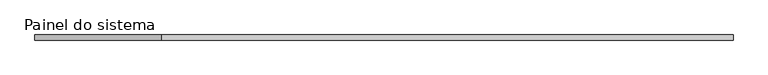
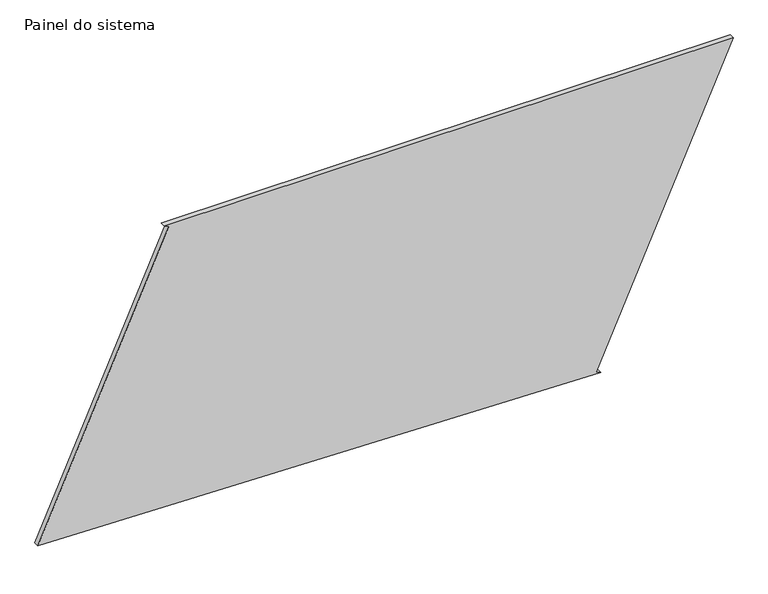
"""IFC4 building model written with IfcOpenShell, lengths in millimetres: plate geometry, Painel do sistema : Envidraçado."""

import ifcopenshell
import ifcopenshell.guid

model = None  # the IFC model being written
_history = None  # IfcOwnerHistory: only IFC2X3 demands one
_inside = {}  # id of a spatial element -> (the spatial element, [elements in it])
_under = {}  # id of a project, library or spatial element -> (it, [spatial elements below it])
_declared = {}  # id of a project -> (the project, [libraries it declares])
_typed = {}  # id of a type object -> (the type object, [elements of that type])
_made_of = {}  # id of a material, layer set ... -> (it, [elements and type objects made of it])


def new_model(schema):
    """Start an empty IFC model of exactly this schema.

    Asked for "IFC4X3", IfcOpenShell would pick the latest addendum, in which some entities
    have other attributes; the version numbers below select the first issue.
    IFC2X3 requires an IfcOwnerHistory on every rooted entity: one is made here for all.
    """
    global model, _history
    if schema == "IFC4X3":
        model = ifcopenshell.file(schema_version=(4, 3, 0, 0))
    else:
        model = ifcopenshell.file(schema=schema)
    _inside.clear()
    _under.clear()
    _declared.clear()
    _typed.clear()
    _made_of.clear()
    _history = None
    if model.schema == "IFC2X3":
        org = make("IfcOrganization", Name="unknown")
        user = make(
            "IfcPersonAndOrganization",
            ThePerson=make("IfcPerson", FamilyName="unknown"),
            TheOrganization=org,
        )
        app = make(
            "IfcApplication",
            ApplicationDeveloper=org,
            Version="unknown",
            ApplicationFullName="unknown",
            ApplicationIdentifier="unknown",
        )
        _history = make(
            "IfcOwnerHistory",
            OwningUser=user,
            OwningApplication=app,
            ChangeAction="ADDED",
            CreationDate=0,
        )
    return model


def make(cls, **values):
    """One entity of the class cls with the attributes given. An attribute that is None is left unset."""
    return model.create_entity(
        cls, **{name: value for name, value in values.items() if value is not None}
    )


def rooted(cls, **values):
    """An entity with a GlobalId (a new one), such as an element, a storey or a relation."""
    return make(cls, GlobalId=ifcopenshell.guid.new(), OwnerHistory=_history, **values)


def si_unit(unit_type, name, prefix=None):
    """IfcSIUnit, for example si_unit("LENGTHUNIT", "METRE", prefix="MILLI")."""
    return make("IfcSIUnit", UnitType=unit_type, Prefix=prefix, Name=name)


def assignment(units):
    """IfcUnitAssignment: the units of a project."""
    return None if units is None else make("IfcUnitAssignment", Units=units)


def point(xyz):
    """IfcCartesianPoint."""
    return None if xyz is None else make("IfcCartesianPoint", Coordinates=xyz)


def direction(xyz):
    """IfcDirection."""
    return None if xyz is None else make("IfcDirection", DirectionRatios=xyz)


def frame(location, z_axis=None, x_axis=None):
    """IfcAxis2Placement3D, a coordinate frame: its origin and axes. An axis left out is left unset."""
    return make(
        "IfcAxis2Placement3D",
        Location=point(location),
        Axis=direction(z_axis),
        RefDirection=direction(x_axis),
    )


def origin():
    """The frame at (0, 0, 0) with its axes left unset."""
    return frame((0.0, 0.0, 0.0))


def place(relative_to, where):
    """IfcLocalPlacement: puts the frame where relative to a parent placement (None: the world)."""
    return make(
        "IfcLocalPlacement", PlacementRelTo=relative_to, RelativePlacement=where
    )


def context(
    kind, dimensions, precision=None, world=None, true_north=None, identifier=None
):
    """IfcGeometricRepresentationContext, for example the 3D "Model" context."""
    return make(
        "IfcGeometricRepresentationContext",
        ContextIdentifier=identifier,
        ContextType=kind,
        CoordinateSpaceDimension=dimensions,
        Precision=precision,
        WorldCoordinateSystem=world,
        TrueNorth=true_north,
    )


def project(units=None, contexts=None):
    """IfcProject with its units and contexts."""
    return rooted(
        "IfcProject",
        Name="project",
        RepresentationContexts=contexts,
        UnitsInContext=assignment(units),
    )


def spatial(cls, under=None, at=None, **own):
    """A site, building, storey or space (cls), placed at a placement, below another one or the project."""
    s = rooted(cls, ObjectPlacement=at, **own)
    if under is not None:
        _under.setdefault(under.id(), (under, []))[1].append(s)
    return s


def polyline(points):
    """IfcPolyline through the points."""
    return make("IfcPolyline", Points=[point(p) for p in points])


def outline(outer, holes=None, kind="AREA"):
    """IfcArbitraryClosedProfileDef: a profile drawn as a closed curve; with holes, ...WithVoids."""
    if holes is None:
        return make("IfcArbitraryClosedProfileDef", ProfileType=kind, OuterCurve=outer)
    return make(
        "IfcArbitraryProfileDefWithVoids",
        ProfileType=kind,
        OuterCurve=outer,
        InnerCurves=holes,
    )


def extrude(swept, where, along, depth):
    """IfcExtrudedAreaSolid: the profile swept, set in the frame where, extruded along a direction by depth."""
    return make(
        "IfcExtrudedAreaSolid",
        SweptArea=swept,
        Position=where,
        ExtrudedDirection=direction(along),
        Depth=depth,
    )


def shape(context_of_items, identifier, shape_type, items):
    """IfcShapeRepresentation: the items that make up one representation, for example the "Body"."""
    return make(
        "IfcShapeRepresentation",
        ContextOfItems=context_of_items,
        RepresentationIdentifier=identifier,
        RepresentationType=shape_type,
        Items=items,
    )


def source(mapping_origin, context_of_items, identifier, shape_type, items):
    """IfcRepresentationMap: a shape defined once, which mapped items show again and again."""
    return make(
        "IfcRepresentationMap",
        MappingOrigin=mapping_origin,
        MappedRepresentation=shape(context_of_items, identifier, shape_type, items),
    )


def transform(
    local_origin,
    x_axis=None,
    y_axis=None,
    z_axis=None,
    scale=None,
    scale2=None,
    scale3=None,
    uniform=True,
):
    """IfcCartesianTransformationOperator3D, or its non-uniform kind. x_axis, y_axis, z_axis: its Axis1, 2, 3."""
    if uniform:
        return make(
            "IfcCartesianTransformationOperator3D",
            Axis1=direction(x_axis),
            Axis2=direction(y_axis),
            LocalOrigin=point(local_origin),
            Scale=scale,
            Axis3=direction(z_axis),
        )
    return make(
        "IfcCartesianTransformationOperator3DnonUniform",
        Axis1=direction(x_axis),
        Axis2=direction(y_axis),
        LocalOrigin=point(local_origin),
        Scale=scale,
        Axis3=direction(z_axis),
        Scale2=scale2,
        Scale3=scale3,
    )


def mapped(mapping_source, mapping_target):
    """IfcMappedItem: shows the shape of a source again, moved by a transform."""
    return make(
        "IfcMappedItem", MappingSource=mapping_source, MappingTarget=mapping_target
    )


def made_of(thing, what):
    """Note that an element or type object is made of a material, layer set ...; save() writes the relation."""
    if what is not None:
        _made_of.setdefault(what.id(), (what, []))[1].append(thing)
    return thing


def element(
    cls,
    number,
    at=None,
    inside=None,
    cuts=None,
    type_object=None,
    material=None,
    context=None,
    identifier="Body",
    shape_type=None,
    held_by="IfcProductDefinitionShape",
    body=None,
    shapes=None,
    **own,
):
    """One element of the class cls, such as IfcWall. Its Tag is "e" and its number.

    at: its placement. inside: the storey or other place that contains it. cuts: it is an
    opening in that element (IfcRelVoidsElement). A single representation is given by context,
    identifier, shape_type and body (its items); several are given by shapes. held_by: the class
    of the entity that holds the representations. save() writes the other relations.
    """
    e = rooted(cls, Tag="e%d" % number, ObjectPlacement=at, **own)
    if body is not None:
        shapes = [shape(context, identifier, shape_type, body)]
    if shapes is not None:
        e.Representation = make(held_by, Representations=shapes)
    if inside is not None:
        _inside.setdefault(inside.id(), (inside, []))[1].append(e)
    if cuts is not None:
        rooted(
            "IfcRelVoidsElement", RelatingBuildingElement=cuts, RelatedOpeningElement=e
        )
    if type_object is not None:
        _typed.setdefault(type_object.id(), (type_object, []))[1].append(e)
    return made_of(e, material)


def aggregate(whole, parts):
    """IfcRelAggregates: a whole, such as a stair, and the parts it consists of."""
    return rooted("IfcRelAggregates", RelatingObject=whole, RelatedObjects=parts)


def save(model, path):
    """Write the relations noted so far, then the file.

    IfcRelAggregates (storeys below a building ...), IfcRelContainedInSpatialStructure (elements
    in a storey), IfcRelDefinesByType, IfcRelAssociatesMaterial and IfcRelDeclares: one each for
    every whole, place, type object, material and project.
    """
    for whole, parts in _under.values():
        aggregate(whole, parts)
    for where, things in _inside.values():
        rooted(
            "IfcRelContainedInSpatialStructure",
            RelatedElements=things,
            RelatingStructure=where,
        )
    for kind, things in _typed.values():
        rooted("IfcRelDefinesByType", RelatedObjects=things, RelatingType=kind)
    for what, things in _made_of.values():
        rooted("IfcRelAssociatesMaterial", RelatedObjects=things, RelatingMaterial=what)
    for by, libraries in _declared.values():
        rooted("IfcRelDeclares", RelatingContext=by, RelatedDefinitions=libraries)
    model.write(path)


def painel_do_sistema_fa9aa4a1(model_context):
    return source(origin(), model_context, "Body", "SweptSolid", [
        extrude(outline(polyline([(0.0, 1056.0772863), (10.2299965, 1033.2661668), (1510.0669756, 1705.8910743), (1510.0669756, -1086.2000189), (1499.836979, -1063.3888995), (67.1684736, -1705.8910743), (0.0, 1056.0772863)])), frame((0.0, 24.5, 0.0), z_axis=(0.0, 1.0, 0.0), x_axis=(0.0, 0.0, 1.0)), (0.0, 0.0, 1.0), 25.0),
    ])


if __name__ == "__main__":
    model = new_model("IFC4")
    model_context = context("Model", 3, world=origin())
    ifc_project = project(units=[si_unit("LENGTHUNIT", "METRE", prefix="MILLI")], contexts=[model_context])
    site = spatial("IfcSite", under=ifc_project)
    building = spatial("IfcBuilding", under=site)
    placement = place(None, origin())
    painel_do_sistema_shape = painel_do_sistema_fa9aa4a1(model_context)
    element("IfcPlate", 1, ObjectType="Painel do sistema : Envidraçado", at=placement, inside=building, context=model_context, shape_type="MappedRepresentation", body=[
        mapped(painel_do_sistema_shape, transform((0.0, 0.0, 0.0), x_axis=(1.0, 0.0, 0.0), y_axis=(0.0, 1.0, 0.0), z_axis=(0.0, 0.0, 1.0))),
    ])
    save(model, "model.ifc")

# Revit data of these elements
# Type "Painel do sistema : Envidraçado"
#   Construction Type Id = "GSP4R"
#   Analytic Construction = "Vidraça única Pilkington 1/8 pol"
#   Visual Light Transmittance = 0.9
#   Solar Heat Gain Coefficient = 0.86
#   Heat Transfer Coefficient (U) = 6.7069 W/(m²·K)
# Element 1 (IfcPlate, "Painel do sistema : Envidraçado")
#   Materials on its faces: "Vidro"
# Materials
#   "Vidro": class "Vidro", colour RGB 0 128 192, transparency 0.9, Description = "Vidro de sílica", Cost = 0
